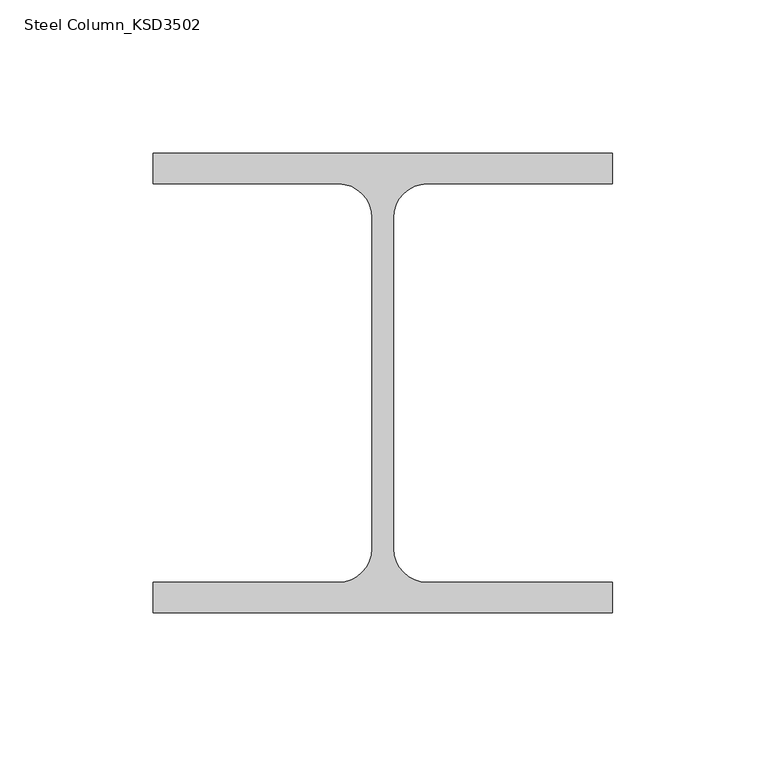
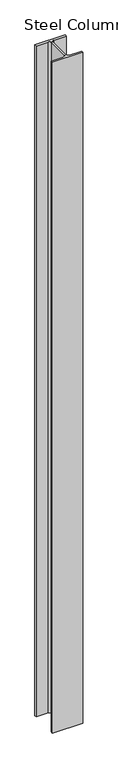
"""IFC4 building model written with IfcOpenShell, lengths in millimetres: column geometry, Steel Column_KSD3502 : H_SC_ASC_H-150×150x7x10."""

from ifc_helpers import new_model, si_unit, point, frame, frame_2d, origin, place, context, project, spatial, polyline, circle_curve, trimmed, segment, composite_curve, outline, extrude, source, transform, mapped, element, save


def steel_column_ksd3502_aafab9da(model_context):
    return source(origin(), model_context, "Body", "SweptSolid", [
        extrude(outline(composite_curve([segment(polyline([(75.0, 75.0), (75.0, 65.0), (14.5, 65.0)]), True, "CONTINUOUS"), segment(trimmed(circle_curve(frame_2d((14.5, 54.0)), 11.0), [point((14.5, 65.0))], [point((3.5, 54.0))], True, "CARTESIAN"), True, "CONTINUOUS"), segment(polyline([(3.5, 54.0), (3.5, -54.0)]), True, "CONTINUOUS"), segment(trimmed(circle_curve(frame_2d((14.5, -54.0)), 11.0), [point((3.5, -54.0))], [point((14.5, -65.0))], True, "CARTESIAN"), True, "CONTINUOUS"), segment(polyline([(14.5, -65.0), (75.0, -65.0), (75.0, -75.0), (-75.0, -75.0), (-75.0, -65.0), (-14.5, -65.0)]), True, "CONTINUOUS"), segment(trimmed(circle_curve(frame_2d((-14.5, -54.0)), 11.0), [point((-14.5, -65.0))], [point((-3.5, -54.0))], True, "CARTESIAN"), True, "CONTINUOUS"), segment(polyline([(-3.5, -54.0), (-3.5, 54.0)]), True, "CONTINUOUS"), segment(trimmed(circle_curve(frame_2d((-14.5, 54.0)), 11.0), [point((-3.5, 54.0))], [point((-14.5, 65.0))], True, "CARTESIAN"), True, "CONTINUOUS"), segment(polyline([(-14.5, 65.0), (-75.0, 65.0), (-75.0, 75.0), (75.0, 75.0)]), True, "CONTINUOUS")], self_intersect=False)), frame((0.0, 0.0, 4449.9720055), z_axis=(0.0, 0.0, 1.0), x_axis=(1.0, 0.0, 0.0)), (0.0, 0.0, 1.0), 3510.0),
    ])


if __name__ == "__main__":
    model = new_model("IFC4")
    model_context = context("Model", 3, world=origin())
    ifc_project = project(units=[si_unit("LENGTHUNIT", "METRE", prefix="MILLI")], contexts=[model_context])
    site = spatial("IfcSite", under=ifc_project)
    building = spatial("IfcBuilding", under=site)
    placement = place(None, origin())
    steel_column_ksd3502_shape = steel_column_ksd3502_aafab9da(model_context)
    element("IfcColumn", 1, ObjectType="Steel Column_KSD3502 : H_SC_ASC_H-150×150x7x10", at=placement, inside=building, context=model_context, shape_type="MappedRepresentation", body=[
        mapped(steel_column_ksd3502_shape, transform((0.0, 0.0, 0.0), x_axis=(1.0, 0.0, 0.0), y_axis=(0.0, 1.0, 0.0), z_axis=(0.0, 0.0, 1.0))),
    ])
    save(model, "model.ifc")

# Revit data of these elements
# Type "Steel Column_KSD3502 : H_SC_ASC_H-150×150x7x10"
#   Width = 15.0 cm
#   Web Thickness = 0.7 cm
#   Web Fillet = 1.1 cm
#   Warping Constant = 27562.5 cm⁶
#   Torsional Moment of Inertia = 11.6007 cm⁴
#   Section Area = 40.14 cm²
#   Plastic Modulus weak axis = 115.0 cm³
#   Plastic Modulus strong axis = 246.0 cm³
#   Perimeter = 1.27 m²/m
#   Nominal Weight = 31.50 kgf/m
#   Moment of Inertia weak axis = 563.00 cm⁴
#   Moment of Inertia strong axis = 1640.00 cm⁴
#   Height = 15.0 cm
#   Flange Thickness = 1.0 cm
#   Elastic Modulus weak axis = 75.1 cm³
#   Elastic Modulus strong axis = 219.0 cm³
#   Centroid Vertical = 7.5 cm
#   Centroid Horizontal = 7.5 cm
#   Bolt Spacing = 13.97 cm
#   Structural Material [instance default] = Steel, 45-345
#   Section Name Key = ""
#   Assembly Code = ""
# Element 1 (IfcColumn, "Steel Column_KSD3502 : H_SC_ASC_H-150×150x7x10")
#   Structural Material = none
# Materials
#   "Steel, 45-345": class "Metal", colour RGB 189 187 185, transparency 0, Description = "Steel 345 MPa", Cost = 0
